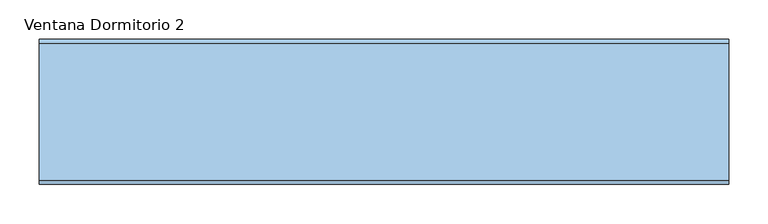
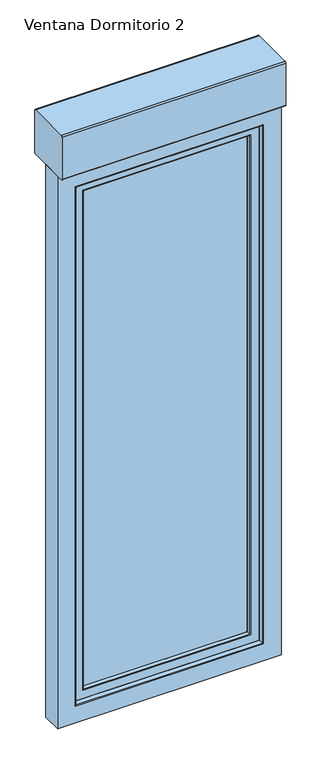
"""IFC4 building model written with IfcOpenShell, lengths in millimetres: window geometry, 2019_ES_Ventana_Replus_re80pvc301_10100_box_1-Hoja_con-Compacto : Ventana Dormitorio 2."""

from ifc_helpers import new_model, si_unit, point, frame, frame_2d, origin, place, context, project, spatial, polyline, circle_curve, ellipse_curve, trimmed, segment, composite_curve, outline, extrude, source, transform, mapped, element, save
from ifc_brep_helpers import plane_surface, cylinder_surface, advanced_brep


def ventana_dormitorio_2_6f2e6c36(model_context):
    return source(origin(), model_context, "Body", "SolidModel", [
        extrude(outline(composite_curve([segment(trimmed(circle_curve(frame_2d((-55.0, 3115.0)), 5.0), [point((-55.0, 3110.0))], [point((-60.0, 3115.0))], False, "CARTESIAN"), True, "CONTINUOUS"), segment(polyline([(-60.0, 3115.0), (-60.0, 3290.0)]), True, "CONTINUOUS"), segment(trimmed(circle_curve(frame_2d((-55.0, 3290.0)), 5.0), [point((-60.0, 3290.0))], [point((-55.0, 3295.0))], False, "CARTESIAN"), True, "CONTINUOUS"), segment(polyline([(-55.0, 3295.0), (120.0, 3295.0)]), True, "CONTINUOUS"), segment(trimmed(circle_curve(frame_2d((120.0, 3290.0)), 5.0), [point((120.0, 3295.0))], [point((125.0, 3290.0))], False, "CARTESIAN"), True, "CONTINUOUS"), segment(polyline([(125.0, 3290.0), (125.0, 3115.0)]), True, "CONTINUOUS"), segment(trimmed(circle_curve(frame_2d((120.0, 3115.0)), 5.0), [point((125.0, 3115.0))], [point((120.0, 3110.0))], False, "CARTESIAN"), True, "CONTINUOUS"), segment(polyline([(120.0, 3110.0), (-55.0, 3110.0)]), True, "CONTINUOUS")], self_intersect=False)), frame((-440.0, 0.0, 0.0), z_axis=(1.0, 0.0, 0.0), x_axis=(0.0, 1.0, 0.0)), (0.0, 0.0, 1.0), 880.0),
        extrude(outline(polyline([(78.4999991, 1470.0), (118.4999991, 1470.0), (118.4999991, 1360.0), (98.4999991, 1360.0), (98.4999991, 1450.0), (78.4999991, 1450.0), (78.4999991, 1470.0)])), frame((-374.1999993, 0.0, 0.0), z_axis=(1.0, 0.0, 0.0), x_axis=(0.0, 1.0, 0.0)), (0.0, 0.0, 1.0), 12.0),
        extrude(outline(polyline([(-353.9687607, 78.4999991), (-353.9687607, 68.4999991), (-382.4312378, 68.4999991), (-382.4312378, 78.4999991), (-353.9687607, 78.4999991)])), frame((0.0, 0.0, 1435.217127), z_axis=(0.0, 0.0, 1.0), x_axis=(1.0, 0.0, 0.0)), (0.0, 0.0, 1.0), 49.565746),
        extrude(outline(polyline([(909.8, 337.1999993), (3007.2, 337.1999993), (3007.2, -337.1999993), (909.8, -337.1999993), (909.8, 337.1999993)]), holes=[polyline([(2999.2, 329.1999993), (917.8, 329.1999993), (917.8, -329.1999993), (2999.2, -329.1999993), (2999.2, 329.1999993)])]), frame((0.0, 10.9999999, 0.0), z_axis=(0.0, 1.0, 0.0), x_axis=(0.0, 0.0, 1.0)), (0.0, 0.0, 1.0), 16.0),
        extrude(outline(polyline([(909.8131934, 337.1868058), (3007.1868066, 337.1868058), (3007.1868066, -337.1868058), (909.8131934, -337.1868058), (909.8131934, 337.1868058)]), holes=[polyline([(2999.2, 329.1999993), (917.8, 329.1999993), (917.8, -329.1999993), (2999.2, -329.1999993), (2999.2, 329.1999993)])]), frame((0.0, 31.0000001, 0.0), z_axis=(0.0, 1.0, 0.0), x_axis=(0.0, 0.0, 1.0)), (0.0, 0.0, 1.0), 16.0),
        extrude(outline(polyline([(337.1999993, 6.9999997), (-337.1999993, 6.9999997), (-337.1999993, 10.9999999), (337.1999993, 10.9999999), (337.1999993, 6.9999997)])), frame((0.0, 0.0, 903.7946451), z_axis=(0.0, 0.0, 1.0), x_axis=(1.0, 0.0, 0.0)), (0.0, 0.0, 1.0), 2109.4053549),
        extrude(outline(polyline([(337.1999993, 26.9999999), (-337.1999993, 26.9999999), (-337.1999993, 31.0000001), (337.1999993, 31.0000001), (337.1999993, 26.9999999)])), frame((0.0, 0.0, 903.7946451), z_axis=(0.0, 0.0, 1.0), x_axis=(1.0, 0.0, 0.0)), (0.0, 0.0, 1.0), 2109.4053549),
        extrude(outline(polyline([(337.1999993, 47.0000001), (-337.1999993, 47.0000001), (-337.1999993, 51.0000003), (337.1999993, 51.0000003), (337.1999993, 47.0000001)])), frame((0.0, 0.0, 903.7946451), z_axis=(0.0, 0.0, 1.0), x_axis=(1.0, 0.0, 0.0)), (0.0, 0.0, 1.0), 2109.4053549),
        advanced_brep(
        [(327.2913171, -9.2764571, 2997.2913178), (327.2913171, -9.2764571, 922.7086822), (330.1890946, -11.5, 919.8109047), (330.1890946, -11.5, 3000.1890953), (370.1999993, -11.5, 879.8), (370.1999993, -11.5, 3040.2), (-370.1999993, -11.5, 3040.2), (-370.1999993, -11.5, 879.8), (-330.1890946, -11.5, 919.8109047), (-330.1890946, -11.5, 3000.1890953), (-327.2913171, -9.2764571, 922.7086822), (324.1757968, 2.3508228, 2994.1757976), (324.1757968, 2.3508228, 925.8242024), (-324.1757968, 2.3508228, 925.8242024), (324.6739305, 3.0000033, 2994.6739313), (324.6739305, 3.0000033, 925.3260687), (-324.6739305, 3.0000033, 925.3260687), (331.1999993, 3.0000033, 3001.2), (331.1999993, 3.0000033, 918.8), (-331.1999993, 3.0000033, 918.8), (-331.1999993, 3.0000033, 3001.2), (-324.6739305, 3.0000033, 2994.6739313), (331.1999993, 6.9999997, 3001.2), (331.1999993, 6.9999997, 918.8), (-331.1999993, 6.9999997, 918.8), (351.8162192, 6.9999997, 3021.8162199), (351.8162192, 6.9999997, 898.1837801), (-351.8162192, 6.9999997, 898.1837801), (-351.8162192, 6.9999997, 3021.8162199), (-331.1999993, 6.9999997, 3001.2), (349.1999993, 25.6153717, 3019.2), (349.1999993, 25.6153717, 900.8), (-349.1999993, 25.6153717, 900.8), (349.1999993, 56.4999995, 3019.2), (349.1999993, 56.4999995, 900.8), (-349.1999993, 56.4999995, 900.8), (-349.1999993, 56.4999995, 3019.2), (337.1999993, 56.4999995, 3007.2), (337.1999993, 56.4999995, 912.8), (-337.1999993, 56.4999995, 912.8), (-337.1999993, 56.4999995, 3007.2), (337.1999993, 51.0000003, 3007.2), (337.1999993, 51.0000003, 912.8), (-337.1999993, 51.0000003, 912.8), (-337.1999993, 51.0000003, 3007.2), (326.007687, 51.0000003, 2996.0076877), (326.007687, 51.0000003, 923.9923123), (-326.007687, 51.0000003, 923.9923123), (-326.007687, 51.0000003, 2996.0076877), (325.4940999, 51.6693201, 2995.4941006), (325.4940999, 51.6693201, 924.5058994), (-325.4940999, 51.6693201, 924.5058994), (328.8993918, 64.3780426, 2998.8993925), (328.8993918, 64.3780426, 921.1006075), (-328.8993918, 64.3780426, 921.1006075), (332.6234971, 67.3403297, 3002.6234978), (332.6234971, 67.3403297, 917.3765022), (-332.6234971, 67.3403297, 917.3765022), (345.6488427, 67.7951848, 3015.6488434), (345.6488427, 67.7951848, 904.3511566), (-345.6488427, 67.7951848, 904.3511566), (346.1999993, 67.2629391, 3016.2), (346.1999993, 67.2629391, 903.8), (-346.1999993, 67.2629391, 903.8), (347.4370593, 68.4999991, 3017.43706), (347.4370593, 68.4999991, 902.56294), (-347.4370593, 68.4999991, 902.56294), (400.1999993, 68.4999991, 3070.2), (400.1999993, 68.4999991, 849.8), (-400.1999993, 68.4999991, 849.8), (-400.1999993, 68.4999991, 3070.2), (-347.4370593, 68.4999991, 3017.43706), (403.1999993, 65.4999991, 3073.2), (403.1999993, 65.4999991, 846.8), (-403.1999993, 65.4999991, 846.8), (403.1999993, 50.0, 3073.2), (403.1999993, 50.0, 846.8), (-403.1999993, 50.0, 846.8), (-403.1999993, 50.0, 3073.2), (383.1999993, 50.0, 3053.2), (383.1999993, 50.0, 866.8), (-383.1999993, 50.0, 866.8), (-383.1999993, 50.0, 3053.2), (383.1999993, 11.9999991, 3053.2), (383.1999993, 11.9999991, 866.8), (-383.1999993, 11.9999991, 866.8), (-383.1999993, 11.9999991, 3053.2), (370.1999993, 11.9999991, 3040.2), (370.1999993, 11.9999991, 879.8), (-370.1999993, 11.9999991, 879.8), (-370.1999993, 11.9999991, 3040.2), (-327.2913171, -9.2764571, 2997.2913178), (-324.1757968, 2.3508228, 2994.1757976), (-349.1999993, 25.6153717, 3019.2), (-325.4940999, 51.6693201, 2995.4941006), (-328.8993918, 64.3780426, 2998.8993925), (-332.6234971, 67.3403297, 3002.6234978), (-345.6488427, 67.7951848, 3015.6488434), (-346.1999993, 67.2629391, 3016.2), (-403.1999993, 65.4999991, 3073.2)],
        [
            (0, 1),
            (1, 2, ellipse_curve(frame((330.1890946, -8.5, 919.8109047), z_axis=(0.7071067811865475, 0.0, 0.7071067811865475), x_axis=(-0.7071067811865474, 0.0, 0.7071067811865476)), 4.2426407, 3.0)),
            (2, 3),
            (3, 0, ellipse_curve(frame((330.1890946, -8.5, 3000.1890953), z_axis=(0.7071067811865475, 0.0, -0.7071067811865475), x_axis=(0.7071067811865474, 0.0, 0.7071067811865476)), 4.2426407, 3.0)),
            (4, 5),
            (5, 6),
            (6, 7),
            (7, 4),
            (2, 8),
            (8, 9),
            (9, 3),
            (1, 10),
            (10, 8, ellipse_curve(frame((-330.1890946, -8.5, 919.8109047), z_axis=(0.7071067811865475, 0.0, -0.7071067811865475), x_axis=(0.7071067811865476, 0.0, 0.7071067811865474)), 4.2426407, 3.0)),
            (11, 12),
            (12, 1),
            (0, 11),
            (12, 13),
            (13, 10),
            (14, 15),
            (15, 12, ellipse_curve(frame((324.6739305, 2.4842973, 925.3260687), z_axis=(0.7071067811865475, 0.0, 0.7071067811865475), x_axis=(-0.7071067811865474, 0.0, 0.7071067811865476)), 0.7293184, 0.515706)),
            (11, 14, ellipse_curve(frame((324.6739305, 2.4842973, 2994.6739313), z_axis=(0.7071067811865475, 0.0, -0.7071067811865475), x_axis=(0.7071067811865474, 0.0, 0.7071067811865476)), 0.7293184, 0.515706)),
            (15, 16),
            (16, 13, ellipse_curve(frame((-324.6739305, 2.4842973, 925.3260687), z_axis=(0.7071067811865475, 0.0, -0.7071067811865475), x_axis=(0.7071067811865476, 0.0, 0.7071067811865474)), 0.7293184, 0.515706)),
            (17, 18),
            (18, 19),
            (19, 20),
            (20, 17),
            (14, 21),
            (21, 16),
            (22, 23),
            (23, 18),
            (17, 22),
            (23, 24),
            (24, 19),
            (25, 26),
            (26, 27),
            (27, 28),
            (28, 25),
            (22, 29),
            (29, 24),
            (30, 31),
            (31, 26),
            (25, 30),
            (31, 32),
            (32, 27),
            (33, 34),
            (34, 31),
            (30, 33),
            (34, 35),
            (35, 32),
            (33, 36),
            (36, 35),
            (37, 38),
            (38, 39),
            (39, 40),
            (40, 37),
            (41, 42),
            (42, 38),
            (37, 41),
            (42, 43),
            (43, 39),
            (41, 44),
            (44, 43),
            (45, 46),
            (46, 47),
            (47, 48),
            (48, 45),
            (49, 50),
            (50, 46, ellipse_curve(frame((326.007687, 51.5317048, 923.9923123), z_axis=(0.7071067811865475, 0.0, 0.7071067811865475), x_axis=(-0.7071067811865474, 0.0, 0.7071067811865476)), 0.7519437, 0.5317045)),
            (45, 49, ellipse_curve(frame((326.007687, 51.5317048, 2996.0076877), z_axis=(0.7071067811865475, 0.0, -0.7071067811865475), x_axis=(0.7071067811865474, 0.0, 0.7071067811865476)), 0.7519437, 0.5317045)),
            (50, 51),
            (51, 47, ellipse_curve(frame((-326.007687, 51.5317048, 923.9923123), z_axis=(0.7071067811865475, 0.0, -0.7071067811865475), x_axis=(0.7071067811865476, 0.0, 0.7071067811865474)), 0.7519437, 0.5317045)),
            (52, 53),
            (53, 50),
            (49, 52),
            (53, 54),
            (54, 51),
            (55, 56),
            (56, 53, ellipse_curve(frame((332.7630951, 63.3427664, 917.2369042), z_axis=(0.7071067811865475, 0.0, 0.7071067811865475), x_axis=(-0.7071067811865474, 0.0, 0.7071067811865476)), 5.6568542, 4.0)),
            (52, 55, ellipse_curve(frame((332.7630951, 63.3427664, 3002.7630958), z_axis=(0.7071067811865475, 0.0, -0.7071067811865475), x_axis=(0.7071067811865474, 0.0, 0.7071067811865476)), 5.6568542, 4.0)),
            (56, 57),
            (57, 54, ellipse_curve(frame((-332.7630951, 63.3427664, 917.2369042), z_axis=(0.7071067811865475, 0.0, -0.7071067811865475), x_axis=(0.7071067811865476, 0.0, 0.7071067811865474)), 5.6568542, 4.0)),
            (58, 59),
            (59, 56),
            (55, 58),
            (59, 60),
            (60, 57),
            (61, 62),
            (62, 59, ellipse_curve(frame((345.6674291, 67.2629391, 904.3325701), z_axis=(0.7071067811865475, 0.0, 0.7071067811865475), x_axis=(-0.7071067811865474, 0.0, 0.7071067811865476)), 0.7531679, 0.5325701)),
            (58, 61, ellipse_curve(frame((345.6674291, 67.2629391, 3015.6674299), z_axis=(0.7071067811865475, 0.0, -0.7071067811865475), x_axis=(0.7071067811865474, 0.0, 0.7071067811865476)), 0.7531679, 0.5325701)),
            (62, 63),
            (63, 60, ellipse_curve(frame((-345.6674291, 67.2629391, 904.3325701), z_axis=(0.7071067811865475, 0.0, -0.7071067811865475), x_axis=(0.7071067811865476, 0.0, 0.7071067811865474)), 0.7531679, 0.5325701)),
            (64, 65),
            (65, 62, ellipse_curve(frame((347.4370593, 67.2629391, 902.56294), z_axis=(0.7071067811865475, 0.0, 0.7071067811865475), x_axis=(-0.7071067811865474, 0.0, 0.7071067811865476)), 1.7494671, 1.23706)),
            (61, 64, ellipse_curve(frame((347.4370593, 67.2629391, 3017.43706), z_axis=(0.7071067811865475, 0.0, -0.7071067811865475), x_axis=(0.7071067811865474, 0.0, 0.7071067811865476)), 1.7494671, 1.23706)),
            (65, 66),
            (66, 63, ellipse_curve(frame((-347.4370593, 67.2629391, 902.56294), z_axis=(0.7071067811865475, 0.0, -0.7071067811865475), x_axis=(0.7071067811865476, 0.0, 0.7071067811865474)), 1.7494671, 1.23706)),
            (67, 68),
            (68, 69),
            (69, 70),
            (70, 67),
            (64, 71),
            (71, 66),
            (72, 73),
            (73, 68, ellipse_curve(frame((400.1999993, 65.4999991, 849.8), z_axis=(0.7071067811865475, 0.0, 0.7071067811865475), x_axis=(-0.7071067811865474, 0.0, 0.7071067811865476)), 4.2426407, 3.0)),
            (67, 72, ellipse_curve(frame((400.1999993, 65.4999991, 3070.2), z_axis=(0.7071067811865475, 0.0, -0.7071067811865475), x_axis=(0.7071067811865474, 0.0, 0.7071067811865476)), 4.2426407, 3.0)),
            (73, 74),
            (74, 69, ellipse_curve(frame((-400.1999993, 65.4999991, 849.8), z_axis=(0.7071067811865475, 0.0, -0.7071067811865475), x_axis=(0.7071067811865476, 0.0, 0.7071067811865474)), 4.2426407, 3.0)),
            (75, 76),
            (76, 73),
            (72, 75),
            (76, 77),
            (77, 74),
            (75, 78),
            (78, 77),
            (79, 80),
            (80, 81),
            (81, 82),
            (82, 79),
            (79, 83),
            (83, 84),
            (84, 80),
            (84, 85),
            (85, 81),
            (83, 86),
            (86, 85),
            (87, 88),
            (88, 89),
            (89, 90),
            (90, 87),
            (87, 5),
            (4, 88),
            (7, 89),
            (10, 91),
            (91, 9, ellipse_curve(frame((-330.1890946, -8.5, 3000.1890953), z_axis=(-0.7071067811865475, 0.0, -0.7071067811865475), x_axis=(0.7071067811865474, 0.0, -0.7071067811865476)), 4.2426407, 3.0)),
            (13, 92),
            (92, 91),
            (21, 92, ellipse_curve(frame((-324.6739305, 2.4842973, 2994.6739313), z_axis=(-0.7071067811865475, 0.0, -0.7071067811865475), x_axis=(0.7071067811865474, 0.0, -0.7071067811865476)), 0.7293184, 0.515706)),
            (29, 20),
            (32, 93),
            (93, 28),
            (36, 93),
            (44, 40),
            (51, 94),
            (94, 48, ellipse_curve(frame((-326.007687, 51.5317048, 2996.0076877), z_axis=(-0.7071067811865475, 0.0, -0.7071067811865475), x_axis=(0.7071067811865474, 0.0, -0.7071067811865476)), 0.7519437, 0.5317045)),
            (54, 95),
            (95, 94),
            (57, 96),
            (96, 95, ellipse_curve(frame((-332.7630951, 63.3427664, 3002.7630958), z_axis=(-0.7071067811865475, 0.0, -0.7071067811865475), x_axis=(0.7071067811865474, 0.0, -0.7071067811865476)), 5.6568542, 4.0)),
            (60, 97),
            (97, 96),
            (63, 98),
            (98, 97, ellipse_curve(frame((-345.6674291, 67.2629391, 3015.6674299), z_axis=(-0.7071067811865475, 0.0, -0.7071067811865475), x_axis=(0.7071067811865474, 0.0, -0.7071067811865476)), 0.7531679, 0.5325701)),
            (71, 98, ellipse_curve(frame((-347.4370593, 67.2629391, 3017.43706), z_axis=(-0.7071067811865475, 0.0, -0.7071067811865475), x_axis=(0.7071067811865474, 0.0, -0.7071067811865476)), 1.7494671, 1.23706)),
            (74, 99),
            (99, 70, ellipse_curve(frame((-400.1999993, 65.4999991, 3070.2), z_axis=(-0.7071067811865475, 0.0, -0.7071067811865475), x_axis=(0.7071067811865474, 0.0, -0.7071067811865476)), 4.2426407, 3.0)),
            (78, 99),
            (86, 82),
            (6, 90),
            (91, 0),
            (92, 11),
            (93, 30),
            (94, 49),
            (95, 52),
            (96, 55),
            (97, 58),
            (98, 61),
            (99, 72),
        ],
        [
            cylinder_surface(frame((330.1890946, -8.5, 3073.2), z_axis=(0.0, 0.0, 1.0), x_axis=(-1.0, 0.0, 0.0)), 3.0),
            plane_surface(frame((-370.1999993, -11.5, 3040.2), z_axis=(0.0, -1.0, 0.0), x_axis=(1.0, 0.0, 0.0))),
            cylinder_surface(frame((403.1999993, -8.5, 919.8109047), z_axis=(1.0, 0.0, 0.0), x_axis=(0.0, 0.0, 1.0)), 3.0),
            plane_surface(frame((327.2913171, -9.2764571, 2997.2913178), z_axis=(-0.9659258263570549, -0.25881904484879154, 0.0), x_axis=(0.0, 0.0, -1.0))),
            plane_surface(frame((327.2913171, -9.2764571, 922.7086822), z_axis=(0.0, -0.2588190448487884, 0.9659258263570558), x_axis=(-1.0, 0.0, 0.0))),
            cylinder_surface(frame((324.6739305, 2.4842973, 3073.2), z_axis=(0.0, 0.0, 1.0), x_axis=(-1.0, 0.0, 0.0)), 0.515706),
            cylinder_surface(frame((403.1999993, 2.4842973, 925.3260687), z_axis=(1.0, 0.0, 0.0), x_axis=(0.0, 0.0, 1.0)), 0.515706),
            plane_surface(frame((-324.6739305, 3.0000033, 2994.6739313), z_axis=(0.0, 1.0, 0.0), x_axis=(1.0, 0.0, 0.0))),
            plane_surface(frame((331.1999993, 3.0000033, 3001.2), z_axis=(-1.0, 0.0, 0.0), x_axis=(0.0, 0.0, -1.0))),
            plane_surface(frame((331.1999993, 3.0000033, 918.8), z_axis=(0.0, 0.0, 1.0), x_axis=(-1.0, 0.0, 0.0))),
            plane_surface(frame((-331.1999993, 6.9999997, 3001.2), z_axis=(0.0, 1.0, 0.0), x_axis=(1.0, 0.0, 0.0))),
            plane_surface(frame((351.8162192, 6.9999997, 3021.8162199), z_axis=(-0.9902680687415736, -0.13917310096004265, 0.0), x_axis=(0.0, 0.0, -1.0))),
            plane_surface(frame((351.8162192, 6.9999997, 898.1837801), z_axis=(0.0, -0.13917310096003946, 0.990268068741574), x_axis=(-1.0, 0.0, 0.0))),
            plane_surface(frame((349.1999993, 25.6153717, 3019.2), z_axis=(-1.0, 0.0, 0.0), x_axis=(0.0, 0.0, -1.0))),
            plane_surface(frame((349.1999993, 25.6153717, 900.8), z_axis=(0.0, 0.0, 1.0), x_axis=(-1.0, 0.0, 0.0))),
            plane_surface(frame((-349.1999993, 56.4999995, 3019.2), z_axis=(0.0, -1.0, 0.0), x_axis=(1.0, 0.0, 0.0))),
            plane_surface(frame((337.1999993, 56.4999995, 3007.2), z_axis=(1.0, 0.0, 0.0), x_axis=(0.0, 0.0, -1.0))),
            plane_surface(frame((337.1999993, 56.4999995, 912.8), z_axis=(0.0, 0.0, -1.0), x_axis=(-1.0, 0.0, 0.0))),
            plane_surface(frame((-337.1999993, 51.0000003, 3007.2), z_axis=(0.0, -1.0, 0.0), x_axis=(1.0, 0.0, 0.0))),
            cylinder_surface(frame((326.007687, 51.5317048, 3073.2), z_axis=(0.0, 0.0, 1.0), x_axis=(-1.0, 0.0, 0.0)), 0.5317045),
            cylinder_surface(frame((403.1999993, 51.5317048, 923.9923123), z_axis=(1.0, 0.0, 0.0), x_axis=(0.0, 0.0, 1.0)), 0.5317045),
            plane_surface(frame((325.4940999, 51.6693201, 2995.4941006), z_axis=(-0.9659258262890665, 0.2588190451025274, 0.0), x_axis=(0.0, 0.0, -1.0))),
            plane_surface(frame((325.4940999, 51.6693201, 924.5058994), z_axis=(0.0, 0.25881904510253056, 0.9659258262890658), x_axis=(-1.0, 0.0, 0.0))),
            cylinder_surface(frame((332.7630951, 63.3427664, 3073.2), z_axis=(0.0, 0.0, 1.0), x_axis=(-1.0, 0.0, 0.0)), 4.0),
            cylinder_surface(frame((403.1999993, 63.3427664, 917.2369042), z_axis=(1.0, 0.0, 0.0), x_axis=(0.0, 0.0, 1.0)), 4.0),
            plane_surface(frame((332.6234971, 67.3403297, 3002.6234978), z_axis=(-0.034899496702507804, 0.9993908270190955, 0.0), x_axis=(0.0, 0.0, -1.0))),
            plane_surface(frame((332.6234971, 67.3403297, 917.3765022), z_axis=(0.0, 0.9993908270190957, 0.03489949670250458), x_axis=(-1.0, 0.0, 0.0))),
            cylinder_surface(frame((345.6674291, 67.2629391, 3073.2), z_axis=(0.0, 0.0, 1.0), x_axis=(-1.0, 0.0, 0.0)), 0.5325701),
            cylinder_surface(frame((403.1999993, 67.2629391, 904.3325701), z_axis=(1.0, 0.0, 0.0), x_axis=(0.0, 0.0, 1.0)), 0.5325701),
            cylinder_surface(frame((347.4370593, 67.2629391, 3073.2), z_axis=(0.0, 0.0, 1.0), x_axis=(-1.0, 0.0, 0.0)), 1.23706),
            cylinder_surface(frame((403.1999993, 67.2629391, 902.56294), z_axis=(1.0, 0.0, 0.0), x_axis=(0.0, 0.0, 1.0)), 1.23706),
            plane_surface(frame((-347.4370593, 68.4999991, 3017.43706), z_axis=(0.0, 1.0, 0.0), x_axis=(1.0, 0.0, 0.0))),
            cylinder_surface(frame((400.1999993, 65.4999991, 3073.2), z_axis=(0.0, 0.0, 1.0), x_axis=(-1.0, 0.0, 0.0)), 3.0),
            cylinder_surface(frame((403.1999993, 65.4999991, 849.8), z_axis=(1.0, 0.0, 0.0), x_axis=(0.0, 0.0, 1.0)), 3.0),
            plane_surface(frame((403.1999993, 65.4999991, 3073.2), z_axis=(1.0, 0.0, 0.0), x_axis=(0.0, 0.0, -1.0))),
            plane_surface(frame((403.1999993, 65.4999991, 846.8), z_axis=(0.0, 0.0, -1.0), x_axis=(-1.0, 0.0, 0.0))),
            plane_surface(frame((-399.2000019, 50.0, 3069.2000027), z_axis=(0.0, -1.0, 0.0), x_axis=(1.0, 0.0, 0.0))),
            plane_surface(frame((383.1999993, 45.0999991, 3053.2), z_axis=(1.0, 0.0, 0.0), x_axis=(0.0, 0.0, -1.0))),
            plane_surface(frame((383.1999993, 45.0999991, 866.8), z_axis=(0.0, 0.0, -1.0), x_axis=(-1.0, 0.0, 0.0))),
            plane_surface(frame((-375.7000002, 11.9999991, 3045.7000009), z_axis=(0.0, -1.0, 0.0), x_axis=(1.0, 0.0, 0.0))),
            plane_surface(frame((370.1999993, 1.4999991, 3040.2), z_axis=(1.0, 0.0, 0.0), x_axis=(0.0, 0.0, -1.0))),
            plane_surface(frame((370.1999993, 1.4999991, 879.8), z_axis=(0.0, 0.0, -1.0), x_axis=(-1.0, 0.0, 0.0))),
            cylinder_surface(frame((-330.1890946, -8.5, 846.8), z_axis=(0.0, 0.0, -1.0), x_axis=(1.0, 0.0, 0.0)), 3.0),
            plane_surface(frame((-327.2913171, -9.2764571, 922.7086822), z_axis=(0.9659258263570565, -0.25881904484878526, 0.0), x_axis=(0.0, 0.0, 1.0))),
            cylinder_surface(frame((-324.6739305, 2.4842973, 846.8), z_axis=(0.0, 0.0, -1.0), x_axis=(1.0, 0.0, 0.0)), 0.515706),
            plane_surface(frame((-331.1999993, 3.0000033, 918.8), z_axis=(1.0, 0.0, 0.0), x_axis=(0.0, 0.0, 1.0))),
            plane_surface(frame((-351.8162192, 6.9999997, 898.1837801), z_axis=(0.9902680687415745, -0.13917310096003627, 0.0), x_axis=(0.0, 0.0, 1.0))),
            plane_surface(frame((-349.1999993, 25.6153717, 900.8), z_axis=(1.0, 0.0, 0.0), x_axis=(0.0, 0.0, 1.0))),
            plane_surface(frame((-337.1999993, 56.4999995, 912.8), z_axis=(-1.0, 0.0, 0.0), x_axis=(0.0, 0.0, 1.0))),
            cylinder_surface(frame((-326.007687, 51.5317048, 846.8), z_axis=(0.0, 0.0, -1.0), x_axis=(1.0, 0.0, 0.0)), 0.5317045),
            plane_surface(frame((-325.4940999, 51.6693201, 924.5058994), z_axis=(0.9659258262890649, 0.2588190451025337, 0.0), x_axis=(0.0, 0.0, 1.0))),
            cylinder_surface(frame((-332.7630951, 63.3427664, 846.8), z_axis=(0.0, 0.0, -1.0), x_axis=(1.0, 0.0, 0.0)), 4.0),
            plane_surface(frame((-332.6234971, 67.3403297, 917.3765022), z_axis=(0.03489949670250135, 0.9993908270190958, 0.0), x_axis=(0.0, 0.0, 1.0))),
            cylinder_surface(frame((-345.6674291, 67.2629391, 846.8), z_axis=(0.0, 0.0, -1.0), x_axis=(1.0, 0.0, 0.0)), 0.5325701),
            cylinder_surface(frame((-347.4370593, 67.2629391, 846.8), z_axis=(0.0, 0.0, -1.0), x_axis=(1.0, 0.0, 0.0)), 1.23706),
            cylinder_surface(frame((-400.1999993, 65.4999991, 846.8), z_axis=(0.0, 0.0, -1.0), x_axis=(1.0, 0.0, 0.0)), 3.0),
            plane_surface(frame((-403.1999993, 65.4999991, 846.8), z_axis=(-1.0, 0.0, 0.0), x_axis=(0.0, 0.0, 1.0))),
            plane_surface(frame((-383.1999993, 45.0999991, 866.8), z_axis=(-1.0, 0.0, 0.0), x_axis=(0.0, 0.0, 1.0))),
            plane_surface(frame((-370.1999993, 1.4999991, 879.8), z_axis=(-1.0, 0.0, 0.0), x_axis=(0.0, 0.0, 1.0))),
            cylinder_surface(frame((-403.1999993, -8.5, 3000.1890953), z_axis=(-1.0, 0.0, 0.0), x_axis=(0.0, 0.0, -1.0)), 3.0),
            plane_surface(frame((-327.2913171, -9.2764571, 2997.2913178), z_axis=(0.0, -0.2588190448487884, -0.9659258263570557), x_axis=(1.0, 0.0, 0.0))),
            cylinder_surface(frame((-403.1999993, 2.4842973, 2994.6739313), z_axis=(-1.0, 0.0, 0.0), x_axis=(0.0, 0.0, -1.0)), 0.515706),
            plane_surface(frame((-331.1999993, 3.0000033, 3001.2), z_axis=(0.0, 0.0, -1.0), x_axis=(1.0, 0.0, 0.0))),
            plane_surface(frame((-351.8162192, 6.9999997, 3021.8162199), z_axis=(0.0, -0.13917310096003946, -0.990268068741574), x_axis=(1.0, 0.0, 0.0))),
            plane_surface(frame((-349.1999993, 25.6153717, 3019.2), z_axis=(0.0, 0.0, -1.0), x_axis=(1.0, 0.0, 0.0))),
            plane_surface(frame((-337.1999993, 56.4999995, 3007.2), z_axis=(0.0, 0.0, 1.0), x_axis=(1.0, 0.0, 0.0))),
            cylinder_surface(frame((-403.1999993, 51.5317048, 2996.0076877), z_axis=(-1.0, 0.0, 0.0), x_axis=(0.0, 0.0, -1.0)), 0.5317045),
            plane_surface(frame((-325.4940999, 51.6693201, 2995.4941006), z_axis=(0.0, 0.25881904510253056, -0.9659258262890658), x_axis=(1.0, 0.0, 0.0))),
            cylinder_surface(frame((-403.1999993, 63.3427664, 3002.7630958), z_axis=(-1.0, 0.0, 0.0), x_axis=(0.0, 0.0, -1.0)), 4.0),
            plane_surface(frame((-332.6234971, 67.3403297, 3002.6234978), z_axis=(0.0, 0.9993908270190957, -0.03489949670250458), x_axis=(1.0, 0.0, 0.0))),
            cylinder_surface(frame((-403.1999993, 67.2629391, 3015.6674299), z_axis=(-1.0, 0.0, 0.0), x_axis=(0.0, 0.0, -1.0)), 0.5325701),
            cylinder_surface(frame((-403.1999993, 67.2629391, 3017.43706), z_axis=(-1.0, 0.0, 0.0), x_axis=(0.0, 0.0, -1.0)), 1.23706),
            cylinder_surface(frame((-403.1999993, 65.4999991, 3070.2), z_axis=(-1.0, 0.0, 0.0), x_axis=(0.0, 0.0, -1.0)), 3.0),
            plane_surface(frame((-403.1999993, 65.4999991, 3073.2), z_axis=(0.0, 0.0, 1.0), x_axis=(1.0, 0.0, 0.0))),
            plane_surface(frame((-383.1999993, 45.0999991, 3053.2), z_axis=(0.0, 0.0, 1.0), x_axis=(1.0, 0.0, 0.0))),
            plane_surface(frame((-370.1999993, 1.4999991, 3040.2), z_axis=(0.0, 0.0, 1.0), x_axis=(1.0, 0.0, 0.0))),
        ],
        [
            (0, [[1, 2, 3, 4]]),
            (1, [[5, 6, 7, 8], [-3, 9, 10, 11]]),
            (2, [[12, 13, -9, -2]]),
            (3, [[14, 15, -1, 16]]),
            (4, [[17, 18, -12, -15]]),
            (5, [[19, 20, -14, 21]]),
            (6, [[22, 23, -17, -20]]),
            (7, [[24, 25, 26, 27], [-19, 28, 29, -22]]),
            (8, [[30, 31, -24, 32]]),
            (9, [[33, 34, -25, -31]]),
            (10, [[35, 36, 37, 38], [-30, 39, 40, -33]]),
            (11, [[41, 42, -35, 43]]),
            (12, [[44, 45, -36, -42]]),
            (13, [[46, 47, -41, 48]]),
            (14, [[49, 50, -44, -47]]),
            (15, [[-46, 51, 52, -49], [53, 54, 55, 56]]),
            (16, [[57, 58, -53, 59]]),
            (17, [[60, 61, -54, -58]]),
            (18, [[-57, 62, 63, -60], [64, 65, 66, 67]]),
            (19, [[68, 69, -64, 70]]),
            (20, [[71, 72, -65, -69]]),
            (21, [[73, 74, -68, 75]]),
            (22, [[76, 77, -71, -74]]),
            (23, [[78, 79, -73, 80]]),
            (24, [[81, 82, -76, -79]]),
            (25, [[83, 84, -78, 85]]),
            (26, [[86, 87, -81, -84]]),
            (27, [[88, 89, -83, 90]]),
            (28, [[91, 92, -86, -89]]),
            (29, [[93, 94, -88, 95]]),
            (30, [[96, 97, -91, -94]]),
            (31, [[98, 99, 100, 101], [-93, 102, 103, -96]]),
            (32, [[104, 105, -98, 106]]),
            (33, [[107, 108, -99, -105]]),
            (34, [[109, 110, -104, 111]]),
            (35, [[112, 113, -107, -110]]),
            (36, [[-109, 114, 115, -112], [116, 117, 118, 119]]),
            (37, [[120, 121, 122, -116]]),
            (38, [[123, 124, -117, -122]]),
            (39, [[-121, 125, 126, -123], [127, 128, 129, 130]]),
            (40, [[131, -5, 132, -127]]),
            (41, [[-8, 133, -128, -132]]),
            (42, [[134, 135, -10, -13]]),
            (43, [[136, 137, -134, -18]]),
            (44, [[-29, 138, -136, -23]]),
            (45, [[-40, 139, -26, -34]]),
            (46, [[140, 141, -37, -45]]),
            (47, [[-52, 142, -140, -50]]),
            (48, [[-63, 143, -55, -61]]),
            (49, [[144, 145, -66, -72]]),
            (50, [[146, 147, -144, -77]]),
            (51, [[148, 149, -146, -82]]),
            (52, [[150, 151, -148, -87]]),
            (53, [[152, 153, -150, -92]]),
            (54, [[-103, 154, -152, -97]]),
            (55, [[155, 156, -100, -108]]),
            (56, [[-115, 157, -155, -113]]),
            (57, [[-126, 158, -118, -124]]),
            (58, [[-7, 159, -129, -133]]),
            (59, [[160, -4, -11, -135]]),
            (60, [[161, -16, -160, -137]]),
            (61, [[-28, -21, -161, -138]]),
            (62, [[-39, -32, -27, -139]]),
            (63, [[162, -43, -38, -141]]),
            (64, [[-51, -48, -162, -142]]),
            (65, [[-62, -59, -56, -143]]),
            (66, [[163, -70, -67, -145]]),
            (67, [[164, -75, -163, -147]]),
            (68, [[165, -80, -164, -149]]),
            (69, [[166, -85, -165, -151]]),
            (70, [[167, -90, -166, -153]]),
            (71, [[-102, -95, -167, -154]]),
            (72, [[168, -106, -101, -156]]),
            (73, [[-114, -111, -168, -157]]),
            (74, [[-125, -120, -119, -158]]),
            (75, [[-6, -131, -130, -159]]),
        ],
    ),
        advanced_brep(
        [(363.2673545, -12.758819, 3033.2673545), (363.2673545, -12.758819, 886.7326455), (367.2913185, -27.7764571, 882.7086815), (367.2913185, -27.7764571, 3037.2913185), (370.189096, -30.0, 879.810904), (370.189096, -30.0, 3040.189096), (-363.2673545, -12.758819, 886.7326455), (-367.2913185, -27.7764571, 882.7086815), (364.2332803, -11.5, 3034.2332803), (364.2332803, -11.5, 885.7667197), (440.0, -30.0, 3110.0), (440.0, -30.0, 810.0), (440.0, 50.0, 810.0), (440.0, 50.0, 3110.0), (-440.0, 50.0, 810.0), (-440.0, 50.0, 3110.0), (396.1999993, 50.0, 853.8000007), (396.1999993, 50.0, 3066.1999993), (-396.1999993, 50.0, 3066.1999993), (-396.1999993, 50.0, 853.8000007), (-440.0, -30.0, 810.0), (-440.0, -30.0, 3110.0), (-370.189096, -30.0, 879.810904), (-370.189096, -30.0, 3040.189096), (376.1891471, 8.0, 3046.1891471), (376.1891471, 8.0, 873.8108529), (376.1891471, -11.5, 873.8108529), (376.1891471, -11.5, 3046.1891471), (-376.1891471, -11.5, 873.8108529), (-376.1891471, -11.5, 3046.1891471), (-364.2332803, -11.5, 3034.2332803), (-364.2332803, -11.5, 885.7667197), (-376.1891471, 8.0, 873.8108529), (395.1999993, 8.0, 3065.1999993), (395.1999993, 8.0, 854.8000007), (-395.1999993, 8.0, 854.8000007), (-395.1999993, 8.0, 3065.1999993), (-376.1891471, 8.0, 3046.1891471), (395.1999993, 49.0, 854.8000007), (395.1999993, 49.0, 3065.1999993), (-395.1999993, 49.0, 854.8000007), (-363.2673545, -12.758819, 3033.2673545), (-367.2913185, -27.7764571, 3037.2913185), (-395.1999993, 49.0, 3065.1999993)],
        [
            (0, 1),
            (1, 2),
            (2, 3),
            (3, 0),
            (2, 4, ellipse_curve(frame((370.189096, -27.0, 879.810904), z_axis=(0.7071067811865475, 0.0, 0.7071067811865475), x_axis=(-0.7071067811865474, 0.0, 0.7071067811865476)), 4.2426407, 3.0)),
            (4, 5),
            (5, 3, ellipse_curve(frame((370.189096, -27.0, 3040.189096), z_axis=(0.7071067811865475, 0.0, -0.7071067811865475), x_axis=(0.7071067811865474, 0.0, 0.7071067811865476)), 4.2426407, 3.0)),
            (1, 6),
            (6, 7),
            (7, 2),
            (8, 9),
            (9, 1, ellipse_curve(frame((364.2332803, -12.5, 885.7667197), z_axis=(0.7071067811865475, 0.0, 0.7071067811865475), x_axis=(-0.7071067811865474, 0.0, 0.7071067811865476)), 1.4142136, 1.0)),
            (0, 8, ellipse_curve(frame((364.2332803, -12.5, 3034.2332803), z_axis=(0.7071067811865475, 0.0, -0.7071067811865475), x_axis=(0.7071067811865474, 0.0, 0.7071067811865476)), 1.4142136, 1.0)),
            (10, 11),
            (11, 12),
            (12, 13),
            (13, 10),
            (12, 14),
            (14, 15),
            (15, 13),
            (16, 17),
            (17, 18),
            (18, 19),
            (19, 16),
            (11, 20),
            (20, 14),
            (10, 21),
            (21, 20),
            (4, 22),
            (22, 23),
            (23, 5),
            (24, 25),
            (25, 26),
            (26, 27),
            (27, 24),
            (26, 28),
            (28, 29),
            (29, 27),
            (8, 30),
            (30, 31),
            (31, 9),
            (25, 32),
            (32, 28),
            (33, 34),
            (34, 35),
            (35, 36),
            (36, 33),
            (24, 37),
            (37, 32),
            (16, 38, ellipse_curve(frame((396.1999993, 49.0, 853.8000007), z_axis=(0.7071067811865475, 0.0, 0.7071067811865475), x_axis=(-0.7071067811865474, 0.0, 0.7071067811865476)), 1.4142136, 1.0)),
            (38, 39),
            (39, 17, ellipse_curve(frame((396.1999993, 49.0, 3066.1999993), z_axis=(0.7071067811865475, 0.0, -0.7071067811865475), x_axis=(0.7071067811865474, 0.0, 0.7071067811865476)), 1.4142136, 1.0)),
            (38, 34),
            (33, 39),
            (19, 40, ellipse_curve(frame((-396.1999993, 49.0, 853.8000007), z_axis=(0.7071067811865475, 0.0, -0.7071067811865475), x_axis=(0.7071067811865476, 0.0, 0.7071067811865474)), 1.4142136, 1.0)),
            (40, 38),
            (31, 6, ellipse_curve(frame((-364.2332803, -12.5, 885.7667197), z_axis=(0.7071067811865475, 0.0, -0.7071067811865475), x_axis=(0.7071067811865476, 0.0, 0.7071067811865474)), 1.4142136, 1.0)),
            (7, 22, ellipse_curve(frame((-370.189096, -27.0, 879.810904), z_axis=(0.7071067811865475, 0.0, -0.7071067811865475), x_axis=(0.7071067811865476, 0.0, 0.7071067811865474)), 4.2426407, 3.0)),
            (6, 41),
            (41, 42),
            (42, 7),
            (21, 15),
            (37, 29),
            (40, 35),
            (18, 43, ellipse_curve(frame((-396.1999993, 49.0, 3066.1999993), z_axis=(-0.7071067811865475, 0.0, -0.7071067811865475), x_axis=(0.7071067811865474, 0.0, -0.7071067811865476)), 1.4142136, 1.0)),
            (43, 40),
            (30, 41, ellipse_curve(frame((-364.2332803, -12.5, 3034.2332803), z_axis=(-0.7071067811865475, 0.0, -0.7071067811865475), x_axis=(0.7071067811865474, 0.0, -0.7071067811865476)), 1.4142136, 1.0)),
            (42, 23, ellipse_curve(frame((-370.189096, -27.0, 3040.189096), z_axis=(-0.7071067811865475, 0.0, -0.7071067811865475), x_axis=(0.7071067811865474, 0.0, -0.7071067811865476)), 4.2426407, 3.0)),
            (43, 36),
            (41, 0),
            (3, 42),
            (39, 43),
        ],
        [
            plane_surface(frame((367.2913185, -27.7764571, 3037.2913185), z_axis=(-0.9659258262890693, -0.2588190451025169, 0.0), x_axis=(0.0, 0.0, -1.0))),
            cylinder_surface(frame((370.189096, -27.0, 3110.0), z_axis=(0.0, 0.0, 1.0), x_axis=(-1.0, 0.0, 0.0)), 3.0),
            plane_surface(frame((367.2913185, -27.7764571, 882.7086815), z_axis=(0.0, -0.2588190451025138, 0.9659258262890702), x_axis=(-1.0, 0.0, 0.0))),
            cylinder_surface(frame((364.2332803, -12.5, 3110.0), z_axis=(0.0, 0.0, 1.0), x_axis=(-1.0, 0.0, 0.0)), 1.0),
            plane_surface(frame((440.0, 50.0, 3110.0), z_axis=(1.0, 0.0, 0.0), x_axis=(0.0, 0.0, -1.0))),
            plane_surface(frame((-396.1999993, 50.0, 3066.1999993), z_axis=(0.0, 1.0, 0.0), x_axis=(1.0, 0.0, 0.0))),
            plane_surface(frame((440.0, 50.0, 810.0), z_axis=(0.0, 0.0, -1.0), x_axis=(-1.0, 0.0, 0.0))),
            plane_surface(frame((-440.0, -30.0, 3110.0), z_axis=(0.0, -1.0, 0.0), x_axis=(1.0, 0.0, 0.0))),
            plane_surface(frame((376.1891471, -11.5, 3046.1891471), z_axis=(-1.0, 0.0, 0.0), x_axis=(0.0, 0.0, -1.0))),
            plane_surface(frame((-364.2332803, -11.5, 3034.2332803), z_axis=(0.0, 1.0, 0.0), x_axis=(1.0, 0.0, 0.0))),
            plane_surface(frame((376.1891471, -11.5, 873.8108529), z_axis=(0.0, 0.0, 1.0), x_axis=(-1.0, 0.0, 0.0))),
            plane_surface(frame((-376.1891471, 8.0, 3046.1891471), z_axis=(0.0, 1.0, 0.0), x_axis=(1.0, 0.0, 0.0))),
            cylinder_surface(frame((396.1999993, 49.0, 3110.0), z_axis=(0.0, 0.0, 1.0), x_axis=(-1.0, 0.0, 0.0)), 1.0),
            plane_surface(frame((395.1999993, 8.0, 3065.1999993), z_axis=(-1.0, 0.0, 0.0), x_axis=(0.0, 0.0, -1.0))),
            cylinder_surface(frame((440.0, 49.0, 853.8000007), z_axis=(1.0, 0.0, 0.0), x_axis=(0.0, 0.0, 1.0)), 1.0),
            cylinder_surface(frame((440.0, -12.5, 885.7667197), z_axis=(1.0, 0.0, 0.0), x_axis=(0.0, 0.0, 1.0)), 1.0),
            cylinder_surface(frame((440.0, -27.0, 879.810904), z_axis=(1.0, 0.0, 0.0), x_axis=(0.0, 0.0, 1.0)), 3.0),
            plane_surface(frame((-367.2913185, -27.7764571, 882.7086815), z_axis=(0.9659258262890711, -0.2588190451025107, 0.0), x_axis=(0.0, 0.0, 1.0))),
            plane_surface(frame((-440.0, 50.0, 810.0), z_axis=(-1.0, 0.0, 0.0), x_axis=(0.0, 0.0, 1.0))),
            plane_surface(frame((-376.1891471, -11.5, 873.8108529), z_axis=(1.0, 0.0, 0.0), x_axis=(0.0, 0.0, 1.0))),
            plane_surface(frame((395.1999993, 8.0, 854.8000007), z_axis=(0.0, 0.0, 1.0), x_axis=(-1.0, 0.0, 0.0))),
            cylinder_surface(frame((-396.1999993, 49.0, 810.0), z_axis=(0.0, 0.0, -1.0), x_axis=(1.0, 0.0, 0.0)), 1.0),
            cylinder_surface(frame((-364.2332803, -12.5, 810.0), z_axis=(0.0, 0.0, -1.0), x_axis=(1.0, 0.0, 0.0)), 1.0),
            cylinder_surface(frame((-370.189096, -27.0, 810.0), z_axis=(0.0, 0.0, -1.0), x_axis=(1.0, 0.0, 0.0)), 3.0),
            plane_surface(frame((-395.1999993, 8.0, 854.8000007), z_axis=(1.0, 0.0, 0.0), x_axis=(0.0, 0.0, 1.0))),
            plane_surface(frame((-367.2913185, -27.7764571, 3037.2913185), z_axis=(0.0, -0.2588190451025138, -0.9659258262890702), x_axis=(1.0, 0.0, 0.0))),
            plane_surface(frame((-440.0, 50.0, 3110.0), z_axis=(0.0, 0.0, 1.0), x_axis=(1.0, 0.0, 0.0))),
            plane_surface(frame((-376.1891471, -11.5, 3046.1891471), z_axis=(0.0, 0.0, -1.0), x_axis=(1.0, 0.0, 0.0))),
            cylinder_surface(frame((-440.0, 49.0, 3066.1999993), z_axis=(-1.0, 0.0, 0.0), x_axis=(0.0, 0.0, -1.0)), 1.0),
            cylinder_surface(frame((-440.0, -12.5, 3034.2332803), z_axis=(-1.0, 0.0, 0.0), x_axis=(0.0, 0.0, -1.0)), 1.0),
            cylinder_surface(frame((-440.0, -27.0, 3040.189096), z_axis=(-1.0, 0.0, 0.0), x_axis=(0.0, 0.0, -1.0)), 3.0),
            plane_surface(frame((-395.1999993, 8.0, 3065.1999993), z_axis=(0.0, 0.0, -1.0), x_axis=(1.0, 0.0, 0.0))),
        ],
        [
            (0, [[1, 2, 3, 4]]),
            (1, [[-3, 5, 6, 7]]),
            (2, [[8, 9, 10, -2]]),
            (3, [[11, 12, -1, 13]]),
            (4, [[14, 15, 16, 17]]),
            (5, [[-16, 18, 19, 20], [21, 22, 23, 24]]),
            (6, [[25, 26, -18, -15]]),
            (7, [[-14, 27, 28, -25], [-6, 29, 30, 31]]),
            (8, [[32, 33, 34, 35]]),
            (9, [[-34, 36, 37, 38], [-11, 39, 40, 41]]),
            (10, [[42, 43, -36, -33]]),
            (11, [[44, 45, 46, 47], [-32, 48, 49, -42]]),
            (12, [[-21, 50, 51, 52]]),
            (13, [[-51, 53, -44, 54]]),
            (14, [[-24, 55, 56, -50]]),
            (15, [[-41, 57, -8, -12]]),
            (16, [[-10, 58, -29, -5]]),
            (17, [[59, 60, 61, -9]]),
            (18, [[-28, 62, -19, -26]]),
            (19, [[-49, 63, -37, -43]]),
            (20, [[-56, 64, -45, -53]]),
            (21, [[-23, 65, 66, -55]]),
            (22, [[-40, 67, -59, -57]]),
            (23, [[-61, 68, -30, -58]]),
            (24, [[-66, 69, -46, -64]]),
            (25, [[70, -4, 71, -60]]),
            (26, [[-27, -17, -20, -62]]),
            (27, [[-48, -35, -38, -63]]),
            (28, [[-22, -52, 72, -65]]),
            (29, [[-39, -13, -70, -67]]),
            (30, [[-71, -7, -31, -68]]),
            (31, [[-72, -54, -47, -69]]),
        ],
    ),
    ])


if __name__ == "__main__":
    model = new_model("IFC4")
    model_context = context("Model", 3, world=origin())
    ifc_project = project(units=[si_unit("LENGTHUNIT", "METRE", prefix="MILLI")], contexts=[model_context])
    site = spatial("IfcSite", under=ifc_project)
    building = spatial("IfcBuilding", under=site)
    placement = place(None, origin())
    ventana_dormitorio_2_shape = ventana_dormitorio_2_6f2e6c36(model_context)
    element("IfcWindow", 1, ObjectType="2019_ES_Ventana_Replus_re80pvc301_10100_box_1-Hoja_con-Compacto : Ventana Dormitorio 2", at=placement, inside=building, context=model_context, shape_type="MappedRepresentation", body=[
        mapped(ventana_dormitorio_2_shape, transform((0.0, 0.0, 0.0), x_axis=(1.0, 0.0, 0.0), y_axis=(0.0, 1.0, 0.0), z_axis=(0.0, 0.0, 1.0))),
    ])
    save(model, "model.ifc")

# Revit data of these elements
# Type "2019_ES_Ventana_Replus_re80pvc301_10100_box_1-Hoja_con-Compacto : Ventana Dormitorio 2"
#   Type Mark = "45"
#   URL = "https://replus.es/"
#   Product data url = "https://bimetica.com/es/objetos-bim-replus-ventana-practicable-oscilobatiente-una-hoja-con-compacto-9540"
#   Product Guid = ""
#   Model = "10100 BOX"
#   Material secondary = "Glass"
#   Material main = "PVC"
#   Manufacturer = "Replus"
#   Keynote = "08500"
#   EAN code = ""
#   Description = "Perfiles de PVC con triple junta (por junta rígida en el marco). Protegiendo de este modo todos los puntos de cierre y proporcionando una junta perimetral completa, con un grosor en el perfil de 3 mm. Vidrio de alta calidad con diferentes posibilidades"
#   Assembly Code = "B2020100"
#   Analytic Construction = "<None>"
#   Ι_Wll Thcknss [instance default] = 20.0 cm
#   Ι_Wdth Cntrl = 88.0 cm
#   Ι_Nst Cntrl [instance default] = 0.0 cm
#   Ι_Hndl Hght Cntrl = 65.0 cm
#   Ι_Hght Cntrl = 230.0 cm
#   Rough Width = 90.0 cm
#   Rough Height = 232.0 cm
#   Retranqueo [instance default] = 0.0 cm
#   I_Lf_Cntrl = 80.64 cm
#   Hueco = 1.0 cm
#   Height = 230.0 cm
#   Default Sill Height = 80.0 cm
#   Width = 88.0 cm
#   Altura de Manilla = 65.0 cm
#   Visibilidad Líneas Apertura - Planta = yes
#   Visibilidad Líneas Apertura - Alzado = yes
#   Exceso Dimensiones = no
#   Edition number = 1
#   Advertencia Dimensión = yes
#   Product Material = PVC - Replus - 9152 - White
#   Wall Closure = (empty or 0)
# Element 1 (IfcWindow, "2019_ES_Ventana_Replus_re80pvc301_10100_box_1-Hoja_con-Compacto : Ventana Dormitorio 2")
#   Ι_Wll Thcknss = 10.0 cm
#   Materials on its faces: "PVC - Replus - 9152 - White", "Rubber - Replus - Black", "Glass - Replus"
# Materials
#   "PVC - Replus - 9152 - White": class "Miscellaneous", colour RGB 174 174 166, transparency 0, Manufacturer = "Replus", Comments = "Rendering appearance not upgraded ", URL = "https://replus.es/", Cost = 0
#   "Rubber - Replus - Black": class "Plastic", colour RGB 63 63 63, transparency 0, Description = "Natural rubber, black", Cost = 0
#   "Glass - Replus": class "Glass", colour RGB 218 227 224, transparency 0.85, Cost = 0
